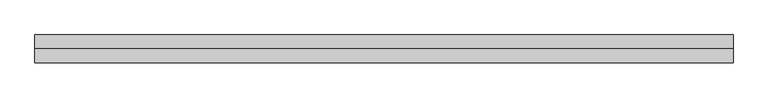
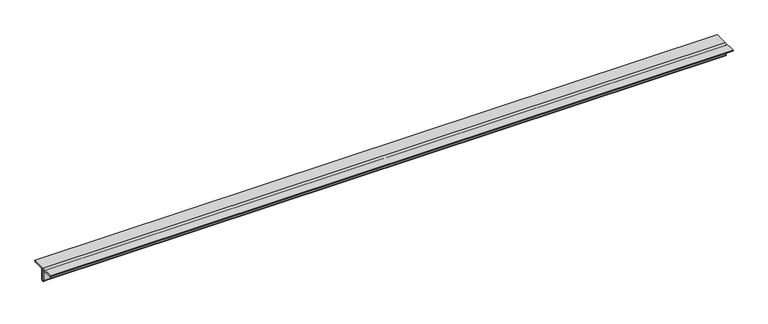
"""IFC4 building model written with IfcOpenShell, lengths in millimetres: member geometry, Steel Framing_2Ls_KS : H_SB_AR_S02_2Ls-100x100x10_VBR1."""

from ifc_helpers import new_model, si_unit, point, frame, frame_2d, origin, place, context, project, spatial, polyline, circle_curve, trimmed, segment, composite_curve, outline, extrude, source, transform, mapped, element, save


def member_a325f419(model_context):
    return source(origin(), model_context, "Body", "SweptSolid", [
        extrude(outline(composite_curve([segment(polyline([(0.0, 28.2), (0.0, -71.8)]), True, "CONTINUOUS"), segment(trimmed(circle_curve(frame_2d((0.0, -61.8)), 10.0), [point((0.0, -71.8))], [point((-10.0, -61.8))], False, "CARTESIAN"), True, "CONTINUOUS"), segment(polyline([(-10.0, -61.8), (-10.0, 8.2)]), True, "CONTINUOUS"), segment(trimmed(circle_curve(frame_2d((-20.0, 8.2)), 10.0), [point((-10.0, 8.2))], [point((-20.0, 18.2))], True, "CARTESIAN"), True, "CONTINUOUS"), segment(polyline([(-20.0, 18.2), (-90.0, 18.2)]), True, "CONTINUOUS"), segment(trimmed(circle_curve(frame_2d((-90.0, 28.2)), 10.0), [point((-90.0, 18.2))], [point((-100.0, 28.2))], False, "CARTESIAN"), True, "CONTINUOUS"), segment(polyline([(-100.0, 28.2), (0.0, 28.2)]), True, "CONTINUOUS")], self_intersect=False)), frame((-2444.561686, 0.0, 0.0), z_axis=(1.0, 0.0, 0.0), x_axis=(0.0, 1.0, 0.0)), (0.0, 0.0, 1.0), 5034.8971694),
        extrude(outline(composite_curve([segment(polyline([(0.0, 28.2), (100.0, 28.2)]), True, "CONTINUOUS"), segment(trimmed(circle_curve(frame_2d((90.0, 28.2)), 10.0), [point((100.0, 28.2))], [point((90.0, 18.2))], False, "CARTESIAN"), True, "CONTINUOUS"), segment(polyline([(90.0, 18.2), (20.0, 18.2)]), True, "CONTINUOUS"), segment(trimmed(circle_curve(frame_2d((20.0, 8.2)), 10.0), [point((20.0, 18.2))], [point((10.0, 8.2))], True, "CARTESIAN"), True, "CONTINUOUS"), segment(polyline([(10.0, 8.2), (10.0, -61.8)]), True, "CONTINUOUS"), segment(trimmed(circle_curve(frame_2d((0.0, -61.8)), 10.0), [point((10.0, -61.8))], [point((0.0, -71.8))], False, "CARTESIAN"), True, "CONTINUOUS"), segment(polyline([(0.0, -71.8), (0.0, 28.2)]), True, "CONTINUOUS")], self_intersect=False)), frame((-2444.561686, 0.0, 0.0), z_axis=(1.0, 0.0, 0.0), x_axis=(0.0, 1.0, 0.0)), (0.0, 0.0, 1.0), 5034.8971694),
    ])


if __name__ == "__main__":
    model = new_model("IFC4")
    model_context = context("Model", 3, world=origin())
    ifc_project = project(units=[si_unit("LENGTHUNIT", "METRE", prefix="MILLI")], contexts=[model_context])
    site = spatial("IfcSite", under=ifc_project)
    building = spatial("IfcBuilding", under=site)
    placement = place(None, origin())
    member_shape = member_a325f419(model_context)
    element("IfcMember", 1, ObjectType="Steel Framing_2Ls_KS : H_SB_AR_S02_2Ls-100x100x10_VBR1", at=placement, inside=building, context=model_context, shape_type="MappedRepresentation", body=[
        mapped(member_shape, transform((0.0, 0.0, 0.0), x_axis=(1.0, 0.0, 0.0), y_axis=(0.0, 1.0, 0.0), z_axis=(0.0, 0.0, 1.0))),
    ])
    save(model, "model.ifc")

# Revit data of these elements
# Type "Steel Framing_2Ls_KS : H_SB_AR_S02_2Ls-100x100x10_VBR1"
#   Type Comments = "MAIN"
#   Type Mark = "VBR1"
#   H_SectionID = "2Ls-100x100x10"
#   Assembly Code = "B10"
#   Legs = "LLBB"
#   H_Ratio for Additional Steel Plate = 0.2
#   W = 0
#   Perimeter = 0.80 m²/m
#   Nominal Weight = 29.80 kgf/m
#   Length [instance default] = 1524 mm
#   Space = 0 mm
#   b = 100 mm
#   d = 100 mm
#   t = 10 mm
#   y = 28.2 mm
#   A = 0.0038 m²
#   Structural Material [instance default] = Steel, 45-345
# Element 1 (IfcMember, "Steel Framing_2Ls_KS : H_SB_AR_S02_2Ls-100x100x10_VBR1")
#   Materials on its faces: "Steel, 45-345"
# Materials
#   "Steel, 45-345": class "Metal", colour RGB 189 187 185, transparency 0, Description = "Steel 345 MPa", Cost = 0
